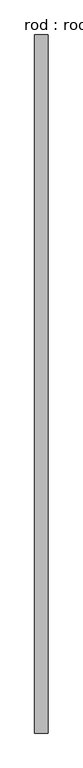
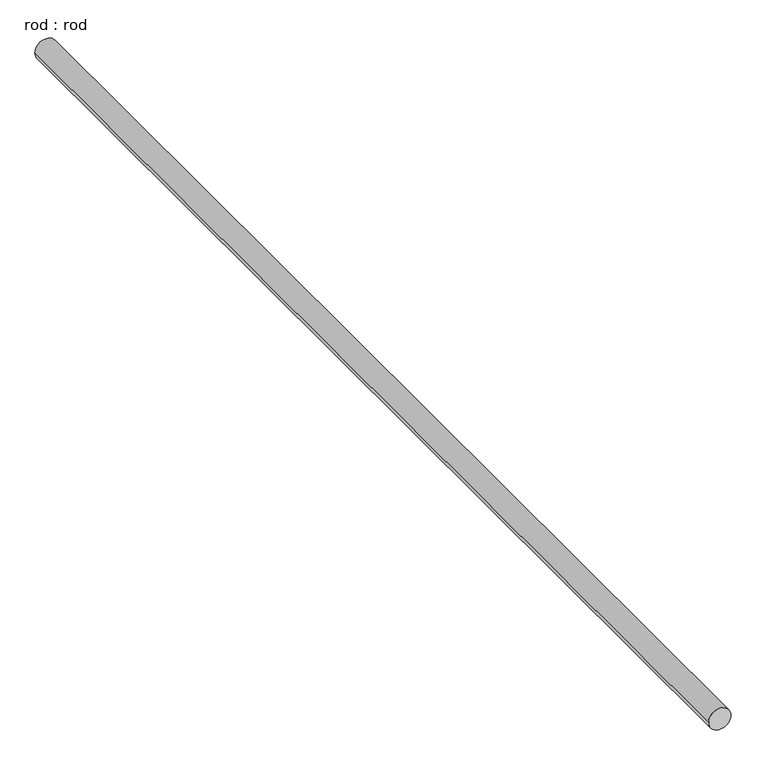
"""IFC4 building model written with IfcOpenShell, lengths in millimetres: proxy geometry, rod : rod."""

from ifc_helpers import new_model, si_unit, point, frame, frame_2d, origin, place, context, project, spatial, circle_curve, trimmed, segment, composite_curve, outline, extrude, source, transform, mapped, element, save


def rod_rod_5a7dcc4c(model_context):
    return source(origin(), model_context, "Body", "SweptSolid", [
        extrude(outline(composite_curve([segment(trimmed(circle_curve(frame_2d((0.0108462, 0.0)), 200.0), [point((0.0108462, 200.0))], [point((0.0108462, -200.0))], False, "CARTESIAN"), True, "CONTINUOUS"), segment(trimmed(circle_curve(frame_2d((0.0108462, 0.0)), 200.0), [point((0.0108462, -200.0))], [point((0.0108462, 200.0))], False, "CARTESIAN"), True, "CONTINUOUS")], self_intersect=False)), frame((0.0, -6378.7884549, 0.0), z_axis=(0.0, 1.0, 0.0), x_axis=(0.0, 0.0, 1.0)), (0.0, 0.0, 1.0), 20943.0341406),
    ])


if __name__ == "__main__":
    model = new_model("IFC4")
    model_context = context("Model", 3, world=origin())
    ifc_project = project(units=[si_unit("LENGTHUNIT", "METRE", prefix="MILLI")], contexts=[model_context])
    site = spatial("IfcSite", under=ifc_project)
    building = spatial("IfcBuilding", under=site)
    placement = place(None, origin())
    rod_rod_shape = rod_rod_5a7dcc4c(model_context)
    element("IfcBuildingElementProxy", 1, Name="rod : rod", ObjectType="rod : rod", at=placement, inside=building, context=model_context, shape_type="MappedRepresentation", body=[
        mapped(rod_rod_shape, transform((0.0, 0.0, 0.0), x_axis=(1.0, 0.0, 0.0), y_axis=(0.0, 1.0, 0.0), z_axis=(0.0, 0.0, 1.0))),
    ])
    save(model, "model.ifc")

# Revit data of these elements
# Type "rod : rod"
#   Default Elevation = 0
